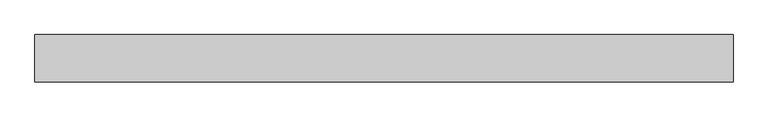
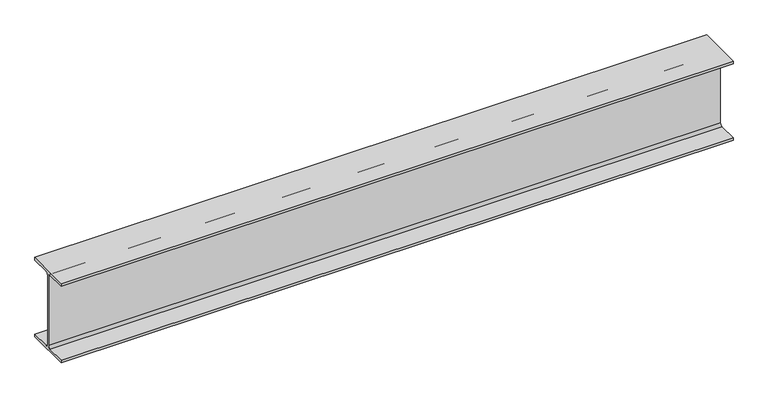
"""IFC4 building model written with IfcOpenShell, lengths in millimetres: beam geometry, Steel Beam_H-KSD3502 : H_SB_ASB_H-200x200x8x12."""

import ifcopenshell
import ifcopenshell.guid

model = None  # the IFC model being written
_history = None  # IfcOwnerHistory: only IFC2X3 demands one
_inside = {}  # id of a spatial element -> (the spatial element, [elements in it])
_under = {}  # id of a project, library or spatial element -> (it, [spatial elements below it])
_declared = {}  # id of a project -> (the project, [libraries it declares])
_typed = {}  # id of a type object -> (the type object, [elements of that type])
_made_of = {}  # id of a material, layer set ... -> (it, [elements and type objects made of it])


def new_model(schema):
    """Start an empty IFC model of exactly this schema.

    Asked for "IFC4X3", IfcOpenShell would pick the latest addendum, in which some entities
    have other attributes; the version numbers below select the first issue.
    IFC2X3 requires an IfcOwnerHistory on every rooted entity: one is made here for all.
    """
    global model, _history
    if schema == "IFC4X3":
        model = ifcopenshell.file(schema_version=(4, 3, 0, 0))
    else:
        model = ifcopenshell.file(schema=schema)
    _inside.clear()
    _under.clear()
    _declared.clear()
    _typed.clear()
    _made_of.clear()
    _history = None
    if model.schema == "IFC2X3":
        org = make("IfcOrganization", Name="unknown")
        user = make(
            "IfcPersonAndOrganization",
            ThePerson=make("IfcPerson", FamilyName="unknown"),
            TheOrganization=org,
        )
        app = make(
            "IfcApplication",
            ApplicationDeveloper=org,
            Version="unknown",
            ApplicationFullName="unknown",
            ApplicationIdentifier="unknown",
        )
        _history = make(
            "IfcOwnerHistory",
            OwningUser=user,
            OwningApplication=app,
            ChangeAction="ADDED",
            CreationDate=0,
        )
    return model


def make(cls, **values):
    """One entity of the class cls with the attributes given. An attribute that is None is left unset."""
    return model.create_entity(
        cls, **{name: value for name, value in values.items() if value is not None}
    )


def rooted(cls, **values):
    """An entity with a GlobalId (a new one), such as an element, a storey or a relation."""
    return make(cls, GlobalId=ifcopenshell.guid.new(), OwnerHistory=_history, **values)


def si_unit(unit_type, name, prefix=None):
    """IfcSIUnit, for example si_unit("LENGTHUNIT", "METRE", prefix="MILLI")."""
    return make("IfcSIUnit", UnitType=unit_type, Prefix=prefix, Name=name)


def assignment(units):
    """IfcUnitAssignment: the units of a project."""
    return None if units is None else make("IfcUnitAssignment", Units=units)


def point(xyz):
    """IfcCartesianPoint."""
    return None if xyz is None else make("IfcCartesianPoint", Coordinates=xyz)


def direction(xyz):
    """IfcDirection."""
    return None if xyz is None else make("IfcDirection", DirectionRatios=xyz)


def frame(location, z_axis=None, x_axis=None):
    """IfcAxis2Placement3D, a coordinate frame: its origin and axes. An axis left out is left unset."""
    return make(
        "IfcAxis2Placement3D",
        Location=point(location),
        Axis=direction(z_axis),
        RefDirection=direction(x_axis),
    )


def frame_2d(location, x_axis=None):
    """IfcAxis2Placement2D, a coordinate frame in the plane: its origin and x axis."""
    return make(
        "IfcAxis2Placement2D", Location=point(location), RefDirection=direction(x_axis)
    )


def origin():
    """The frame at (0, 0, 0) with its axes left unset."""
    return frame((0.0, 0.0, 0.0))


def place(relative_to, where):
    """IfcLocalPlacement: puts the frame where relative to a parent placement (None: the world)."""
    return make(
        "IfcLocalPlacement", PlacementRelTo=relative_to, RelativePlacement=where
    )


def context(
    kind, dimensions, precision=None, world=None, true_north=None, identifier=None
):
    """IfcGeometricRepresentationContext, for example the 3D "Model" context."""
    return make(
        "IfcGeometricRepresentationContext",
        ContextIdentifier=identifier,
        ContextType=kind,
        CoordinateSpaceDimension=dimensions,
        Precision=precision,
        WorldCoordinateSystem=world,
        TrueNorth=true_north,
    )


def project(units=None, contexts=None):
    """IfcProject with its units and contexts."""
    return rooted(
        "IfcProject",
        Name="project",
        RepresentationContexts=contexts,
        UnitsInContext=assignment(units),
    )


def spatial(cls, under=None, at=None, **own):
    """A site, building, storey or space (cls), placed at a placement, below another one or the project."""
    s = rooted(cls, ObjectPlacement=at, **own)
    if under is not None:
        _under.setdefault(under.id(), (under, []))[1].append(s)
    return s


def polyline(points):
    """IfcPolyline through the points."""
    return make("IfcPolyline", Points=[point(p) for p in points])


def circle_curve(where, radius):
    """IfcCircle in the frame where."""
    return make("IfcCircle", Position=where, Radius=radius)


def trimmed(basis, trim1, trim2, sense, master):
    """IfcTrimmedCurve: the piece of a basis curve between two trims."""
    return make(
        "IfcTrimmedCurve",
        BasisCurve=basis,
        Trim1=trim1,
        Trim2=trim2,
        SenseAgreement=sense,
        MasterRepresentation=master,
    )


def segment(curve, same_sense, transition):
    """IfcCompositeCurveSegment."""
    return make(
        "IfcCompositeCurveSegment",
        Transition=transition,
        SameSense=same_sense,
        ParentCurve=curve,
    )


def composite_curve(segments, self_intersect=None):
    """IfcCompositeCurve: segments joined end to end."""
    return make("IfcCompositeCurve", Segments=segments, SelfIntersect=self_intersect)


def outline(outer, holes=None, kind="AREA"):
    """IfcArbitraryClosedProfileDef: a profile drawn as a closed curve; with holes, ...WithVoids."""
    if holes is None:
        return make("IfcArbitraryClosedProfileDef", ProfileType=kind, OuterCurve=outer)
    return make(
        "IfcArbitraryProfileDefWithVoids",
        ProfileType=kind,
        OuterCurve=outer,
        InnerCurves=holes,
    )


def extrude(swept, where, along, depth):
    """IfcExtrudedAreaSolid: the profile swept, set in the frame where, extruded along a direction by depth."""
    return make(
        "IfcExtrudedAreaSolid",
        SweptArea=swept,
        Position=where,
        ExtrudedDirection=direction(along),
        Depth=depth,
    )


def shape(context_of_items, identifier, shape_type, items):
    """IfcShapeRepresentation: the items that make up one representation, for example the "Body"."""
    return make(
        "IfcShapeRepresentation",
        ContextOfItems=context_of_items,
        RepresentationIdentifier=identifier,
        RepresentationType=shape_type,
        Items=items,
    )


def source(mapping_origin, context_of_items, identifier, shape_type, items):
    """IfcRepresentationMap: a shape defined once, which mapped items show again and again."""
    return make(
        "IfcRepresentationMap",
        MappingOrigin=mapping_origin,
        MappedRepresentation=shape(context_of_items, identifier, shape_type, items),
    )


def transform(
    local_origin,
    x_axis=None,
    y_axis=None,
    z_axis=None,
    scale=None,
    scale2=None,
    scale3=None,
    uniform=True,
):
    """IfcCartesianTransformationOperator3D, or its non-uniform kind. x_axis, y_axis, z_axis: its Axis1, 2, 3."""
    if uniform:
        return make(
            "IfcCartesianTransformationOperator3D",
            Axis1=direction(x_axis),
            Axis2=direction(y_axis),
            LocalOrigin=point(local_origin),
            Scale=scale,
            Axis3=direction(z_axis),
        )
    return make(
        "IfcCartesianTransformationOperator3DnonUniform",
        Axis1=direction(x_axis),
        Axis2=direction(y_axis),
        LocalOrigin=point(local_origin),
        Scale=scale,
        Axis3=direction(z_axis),
        Scale2=scale2,
        Scale3=scale3,
    )


def mapped(mapping_source, mapping_target):
    """IfcMappedItem: shows the shape of a source again, moved by a transform."""
    return make(
        "IfcMappedItem", MappingSource=mapping_source, MappingTarget=mapping_target
    )


def made_of(thing, what):
    """Note that an element or type object is made of a material, layer set ...; save() writes the relation."""
    if what is not None:
        _made_of.setdefault(what.id(), (what, []))[1].append(thing)
    return thing


def element(
    cls,
    number,
    at=None,
    inside=None,
    cuts=None,
    type_object=None,
    material=None,
    context=None,
    identifier="Body",
    shape_type=None,
    held_by="IfcProductDefinitionShape",
    body=None,
    shapes=None,
    **own,
):
    """One element of the class cls, such as IfcWall. Its Tag is "e" and its number.

    at: its placement. inside: the storey or other place that contains it. cuts: it is an
    opening in that element (IfcRelVoidsElement). A single representation is given by context,
    identifier, shape_type and body (its items); several are given by shapes. held_by: the class
    of the entity that holds the representations. save() writes the other relations.
    """
    e = rooted(cls, Tag="e%d" % number, ObjectPlacement=at, **own)
    if body is not None:
        shapes = [shape(context, identifier, shape_type, body)]
    if shapes is not None:
        e.Representation = make(held_by, Representations=shapes)
    if inside is not None:
        _inside.setdefault(inside.id(), (inside, []))[1].append(e)
    if cuts is not None:
        rooted(
            "IfcRelVoidsElement", RelatingBuildingElement=cuts, RelatedOpeningElement=e
        )
    if type_object is not None:
        _typed.setdefault(type_object.id(), (type_object, []))[1].append(e)
    return made_of(e, material)


def aggregate(whole, parts):
    """IfcRelAggregates: a whole, such as a stair, and the parts it consists of."""
    return rooted("IfcRelAggregates", RelatingObject=whole, RelatedObjects=parts)


def save(model, path):
    """Write the relations noted so far, then the file.

    IfcRelAggregates (storeys below a building ...), IfcRelContainedInSpatialStructure (elements
    in a storey), IfcRelDefinesByType, IfcRelAssociatesMaterial and IfcRelDeclares: one each for
    every whole, place, type object, material and project.
    """
    for whole, parts in _under.values():
        aggregate(whole, parts)
    for where, things in _inside.values():
        rooted(
            "IfcRelContainedInSpatialStructure",
            RelatedElements=things,
            RelatingStructure=where,
        )
    for kind, things in _typed.values():
        rooted("IfcRelDefinesByType", RelatedObjects=things, RelatingType=kind)
    for what, things in _made_of.values():
        rooted("IfcRelAssociatesMaterial", RelatedObjects=things, RelatingMaterial=what)
    for by, libraries in _declared.values():
        rooted("IfcRelDeclares", RelatingContext=by, RelatedDefinitions=libraries)
    model.write(path)


def beam_3d9c44e8(model_context):
    return source(origin(), model_context, "Body", "SweptSolid", [
        extrude(outline(composite_curve([segment(polyline([(82.5, -141.5), (82.5, -151.7), (-82.5, -151.7), (-82.5, -141.5), (-11.9, -141.5)]), True, "CONTINUOUS"), segment(trimmed(circle_curve(frame_2d((-11.9, -132.6)), 8.9), [point((-11.9, -141.5))], [point((-3.0, -132.6))], True, "CARTESIAN"), True, "CONTINUOUS"), segment(polyline([(-3.0, -132.6), (-3.0, 132.6)]), True, "CONTINUOUS"), segment(trimmed(circle_curve(frame_2d((-11.9, 132.6)), 8.9), [point((-3.0, 132.6))], [point((-11.9, 141.5))], True, "CARTESIAN"), True, "CONTINUOUS"), segment(polyline([(-11.9, 141.5), (-82.5, 141.5), (-82.5, 151.7), (82.5, 151.7), (82.5, 141.5), (11.9, 141.5)]), True, "CONTINUOUS"), segment(trimmed(circle_curve(frame_2d((11.9, 132.6)), 8.9), [point((11.9, 141.5))], [point((3.0, 132.6))], True, "CARTESIAN"), True, "CONTINUOUS"), segment(polyline([(3.0, 132.6), (3.0, -132.6)]), True, "CONTINUOUS"), segment(trimmed(circle_curve(frame_2d((11.9, -132.6)), 8.9), [point((3.0, -132.6))], [point((11.9, -141.5))], True, "CARTESIAN"), True, "CONTINUOUS"), segment(polyline([(11.9, -141.5), (82.5, -141.5)]), True, "CONTINUOUS")], self_intersect=False)), frame((-1238.7267651, 0.0, 0.0), z_axis=(1.0, 0.0, 0.0), x_axis=(0.0, 1.0, 0.0)), (0.0, 0.0, 1.0), 2428.9452569),
    ])


if __name__ == "__main__":
    model = new_model("IFC4")
    model_context = context("Model", 3, world=origin())
    ifc_project = project(units=[si_unit("LENGTHUNIT", "METRE", prefix="MILLI")], contexts=[model_context])
    site = spatial("IfcSite", under=ifc_project)
    building = spatial("IfcBuilding", under=site)
    placement = place(None, origin())
    beam_shape = beam_3d9c44e8(model_context)
    element("IfcBeam", 1, ObjectType="Steel Beam_H-KSD3502 : H_SB_ASB_H-200x200x8x12", at=placement, inside=building, context=model_context, shape_type="MappedRepresentation", body=[
        mapped(beam_shape, transform((0.0, 0.0, 0.0), x_axis=(1.0, 0.0, 0.0), y_axis=(0.0, 1.0, 0.0), z_axis=(0.0, 0.0, 1.0))),
    ])
    save(model, "model.ifc")

# Revit data of these elements
# Type "Steel Beam_H-KSD3502 : H_SB_ASB_H-200x200x8x12"
#   Width = 20.0 cm
#   Web Thickness = 0.8 cm
#   Web Fillet = 1.3 cm
#   Warping Constant = 141376.0 cm⁶
#   Torsional Moment of Inertia = 26.2485 cm⁴
#   Torsional Modulus = 1.0 cm³
#   Section Area = 63.53 cm²
#   Plastic Modulus weak axis = 244.0 cm³
#   Plastic Modulus strong axis = 525.0 cm³
#   Perimeter = 1.16 m²/m
#   Nominal Weight = 49.90 kgf/m
#   Moment of Inertia weak axis = 1600.00 cm⁴
#   Moment of Inertia strong axis = 4720.00 cm⁴
#   Height = 20.0 cm
#   Flange Thickness = 1.2 cm
#   Elastic Modulus weak axis = 160.0 cm³
#   Elastic Modulus strong axis = 472.0 cm³
#   Centroid Vertical = 10.0 cm
#   Centroid Horizontal = 10.0 cm
#   Length [instance default] = 1.5240 m
#   Structural Material [instance default] = Steel, 45-345
#   Assembly Code = ""
# Element 1 (IfcBeam, "Steel Beam_H-KSD3502 : H_SB_ASB_H-200x200x8x12")
#   Structural Material = none
# Materials
#   "Steel, 45-345": class "Metal", colour RGB 189 187 185, transparency 0, Description = "Steel 345 MPa", Cost = 0
